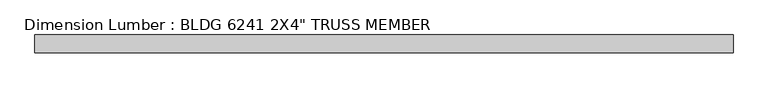
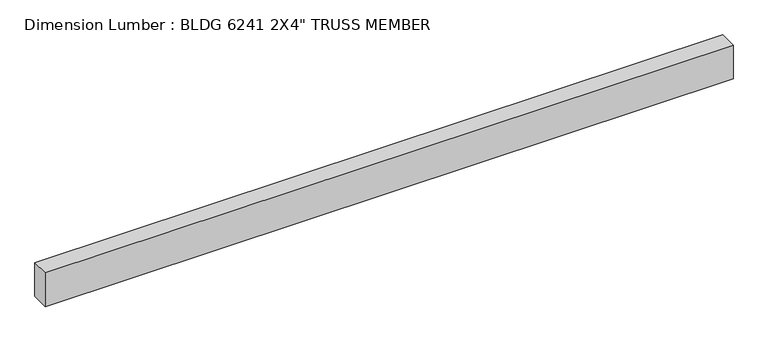
"""IFC4 building model written with IfcOpenShell, lengths in millimetres: beam geometry."""

from ifc_helpers import new_model, si_unit, frame, origin, place, context, project, spatial, polyline, outline, extrude, source, transform, mapped, element, save


def beam_8729cf3f(model_context):
    return source(origin(), model_context, "Body", "SweptSolid", [
        extrude(outline(polyline([(981.075, 25.4), (981.075, -25.4), (-981.075, -25.4), (-981.075, 25.4), (981.075, 25.4)])), frame((0.0, 0.0, -50.8), z_axis=(0.0, 0.0, 1.0), x_axis=(1.0, 0.0, 0.0)), (0.0, 0.0, 1.0), 101.6),
    ])


if __name__ == "__main__":
    model = new_model("IFC4")
    model_context = context("Model", 3, world=origin())
    ifc_project = project(units=[si_unit("LENGTHUNIT", "METRE", prefix="MILLI")], contexts=[model_context])
    site = spatial("IfcSite", under=ifc_project)
    building = spatial("IfcBuilding", under=site)
    placement = place(None, origin())
    beam_shape = beam_8729cf3f(model_context)
    element("IfcBeam", 1, ObjectType="Dimension Lumber : BLDG 6241 2X4\" TRUSS MEMBER", at=placement, inside=building, context=model_context, shape_type="MappedRepresentation", body=[
        mapped(beam_shape, transform((0.0, 0.0, 0.0), x_axis=(1.0, 0.0, 0.0), y_axis=(0.0, 1.0, 0.0), z_axis=(0.0, 0.0, 1.0))),
    ])
    save(model, "model.ifc")

# Revit data of these elements
# Type "Dimension Lumber : BLDG 6241 2X4\" TRUSS MEMBER"
#   Assembly Code = "B10"
#   A = 0.273472 SF
#   Length [instance default] = 5' - 0"
#   b = 0' - 2"
#   d = 0' - 4"
#   Structural Material [instance default] = Softwood, Lumber
# Element 1 (IfcBeam, "Dimension Lumber : BLDG 6241 2X4\" TRUSS MEMBER")
#   Materials on its faces: "Softwood, Lumber"
# Materials
#   "Softwood, Lumber": class "Wood", colour RGB 223 192 134, transparency 0, Description = "Pinus Echinata", Cost = 0
